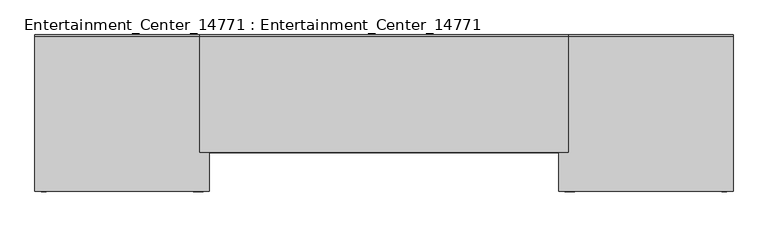
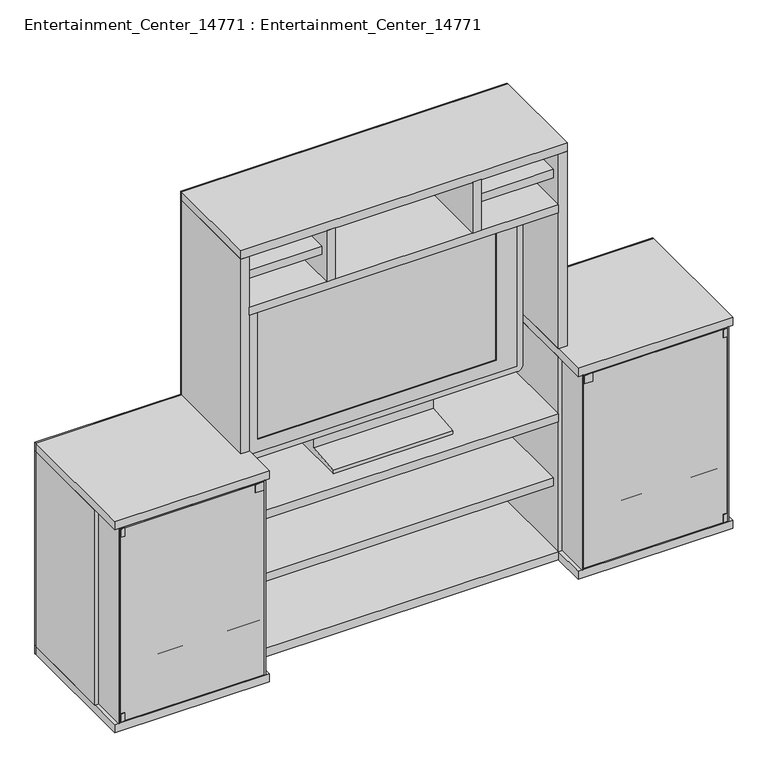
"""IFC4 building model written with IfcOpenShell, lengths in millimetres: furniture geometry, Entertainment_Center_14771 : Entertainment_Center_14771."""

from ifc_helpers import new_model, si_unit, point, frame, frame_2d, origin, origin_with_axes, place, context, project, spatial, polyline, circle_curve, ellipse_curve, trimmed, segment, composite_curve, outline, extrude, faceted_brep, source, transform, mapped, element, save
from ifc_brep_helpers import plane_surface, cylinder_surface, advanced_brep


def entertainment_center_14771_entertainment_center_14771_971748eb(model_context):
    return source(origin(), model_context, "Body", "SolidModel", [
        extrude(outline(polyline([(3.8418696, 537.2), (53.8418696, 537.2), (103.8418696, 457.2), (-96.1581304, 457.2), (-96.1581304, 467.2), (3.8418696, 477.2), (3.8418696, 537.2)])), frame((-176.4901536, 0.0, 0.0), z_axis=(1.0, 0.0, 0.0), x_axis=(0.0, 1.0, 0.0)), (0.0, 0.0, 1.0), 352.9803073),
        faceted_brep([(412.9803073, -14.1581304, 1014.3392838), (-412.9803073, -14.1581304, 1014.3392838), (-412.9803073, -14.1581304, 537.2), (412.9803073, -14.1581304, 537.2), (-352.9803073, -14.1581304, 974.3392838), (352.9803073, -14.1581304, 974.3392838), (352.9803073, -14.1581304, 577.2), (-352.9803073, -14.1581304, 577.2), (412.9803073, 3.8418696, 1014.3392838), (412.9803073, 3.8418696, 537.2), (-412.9803073, 3.8418696, 537.2), (-412.9803073, 3.8418696, 1014.3392838), (-352.9803073, -11.1581304, 974.3392838), (-352.9803073, -11.1581304, 577.2), (352.9803073, -11.1581304, 577.2), (352.9803073, -11.1581304, 974.3392838)], [[[0, 1, 2, 3], [4, 5, 6, 7]], [[8, 9, 10, 11]], [[1, 0, 8, 11]], [[2, 1, 11, 10]], [[3, 2, 10, 9]], [[0, 3, 9, 8]], [[12, 13, 14, 15]], [[12, 15, 5, 4]], [[15, 14, 6, 5]], [[14, 13, 7, 6]], [[13, 12, 4, 7]]]),
        extrude(outline(composite_curve([segment(polyline([(1034.3392838, 417.9803073), (1034.3392838, -417.9803073)]), True, "CONTINUOUS"), segment(trimmed(circle_curve(frame_2d((1019.3392838, -417.9803073)), 15.0), [point((1034.3392838, -417.9803073))], [point((1019.3392838, -432.9803073))], False, "CARTESIAN"), True, "CONTINUOUS"), segment(polyline([(1019.3392838, -432.9803073), (532.2, -432.9803073)]), True, "CONTINUOUS"), segment(trimmed(circle_curve(frame_2d((532.2, -417.9803073)), 15.0), [point((532.2, -432.9803073))], [point((517.2, -417.9803073))], False, "CARTESIAN"), True, "CONTINUOUS"), segment(polyline([(517.2, -417.9803073), (517.2, 417.9803073)]), True, "CONTINUOUS"), segment(trimmed(circle_curve(frame_2d((532.2, 417.9803073)), 15.0), [point((517.2, 417.9803073))], [point((532.2, 432.9803073))], False, "CARTESIAN"), True, "CONTINUOUS"), segment(polyline([(532.2, 432.9803073), (1019.3392838, 432.9803073)]), True, "CONTINUOUS"), segment(trimmed(circle_curve(frame_2d((1019.3392838, 417.9803073)), 15.0), [point((1019.3392838, 432.9803073))], [point((1034.3392838, 417.9803073))], False, "CARTESIAN"), True, "CONTINUOUS")], self_intersect=False), holes=[polyline([(1014.3392838, 412.9803073), (537.2, 412.9803073), (537.2, -412.9803073), (1014.3392838, -412.9803073), (1014.3392838, 412.9803073)])]), frame((0.0, -11.1581304, 0.0), z_axis=(0.0, 1.0, 0.0), x_axis=(0.0, 0.0, 1.0)), (0.0, 0.0, 1.0), 15.0),
        advanced_brep(
        [(-412.9803073, 3.8418696, 537.2), (412.9803073, 3.8418696, 537.2), (412.9803073, 3.8418696, 1014.3392838), (-412.9803073, 3.8418696, 1014.3392838), (302.9803073, 113.8418696, 537.2), (-302.9803073, 113.8418696, 537.2), (-302.9803073, 113.8418696, 904.3392838), (302.9803073, 113.8418696, 904.3392838)],
        [
            (0, 1),
            (1, 2),
            (2, 3),
            (3, 0),
            (4, 5),
            (5, 6),
            (6, 7),
            (7, 4),
            (0, 5, circle_curve(frame((-302.9803073, 3.8418696, 537.2), z_axis=(0.0, 0.0, -1.0), x_axis=(-1.0, 0.0, 0.0)), 110.0)),
            (4, 1, circle_curve(frame((302.9803073, 3.8418696, 537.2), z_axis=(0.0, 0.0, -1.0), x_axis=(1.0, 0.0, 0.0)), 110.0)),
            (7, 2, ellipse_curve(frame((302.9803073, 3.8418696, 904.3392838), z_axis=(0.7071067811865475, 0.0, -0.7071067811865475), x_axis=(0.7071067811865474, 0.0, 0.7071067811865476)), 155.5634919, 110.0)),
            (6, 3, ellipse_curve(frame((-302.9803073, 3.8418696, 904.3392838), z_axis=(0.7071067811865475, 0.0, 0.7071067811865475), x_axis=(-0.7071067811865476, 0.0, 0.7071067811865474)), 155.5634919, 110.0)),
        ],
        [
            plane_surface(frame((-412.9803073, 3.8418696, 1014.3392838), z_axis=(0.0, -1.0, 0.0), x_axis=(-1.0, 0.0, 0.0))),
            plane_surface(frame((-412.9803073, 113.8418696, 1014.3392838), z_axis=(0.0, 1.0, 0.0), x_axis=(1.0, 0.0, 0.0))),
            plane_surface(frame((-412.9803073, 3.8418696, 537.2), z_axis=(0.0, 0.0, -1.0), x_axis=(0.0, 1.0, 0.0))),
            cylinder_surface(frame((302.9803073, 3.8418696, 537.2), z_axis=(0.0, 0.0, 1.0), x_axis=(1.0, 0.0, 0.0)), 110.0),
            cylinder_surface(frame((412.9803073, 3.8418696, 904.3392838), z_axis=(-1.0, 0.0, 0.0), x_axis=(0.0, 0.0, 1.0)), 110.0),
            cylinder_surface(frame((-302.9803073, 3.8418696, 1014.3392838), z_axis=(0.0, 0.0, -1.0), x_axis=(-1.0, 0.0, 0.0)), 110.0),
        ],
        [
            (0, [[1, 2, 3, 4]]),
            (1, [[5, 6, 7, 8]]),
            (2, [[-1, 9, -5, 10]]),
            (3, [[11, -2, -10, -8]]),
            (4, [[-11, -7, 12, -3]]),
            (5, [[-12, -6, -9, -4]]),
        ],
    ),
        extrude(outline(polyline([(468.3125, -254.0), (468.3125, -152.4), (471.4875, -152.4), (471.4875, -254.0), (468.3125, -254.0)])), frame((0.0, 0.0, 25.4), z_axis=(0.0, 0.0, 1.0), x_axis=(1.0, 0.0, 0.0)), (0.0, 0.0, 1.0), 609.6),
        extrude(outline(polyline([(474.0377403, -254.8079035), (474.0377403, -253.9978359), (499.2974238, -253.9978359), (499.2974238, -254.8079035), (474.0377403, -254.8079035)])), frame((0.0, 0.0, 606.4088319), z_axis=(0.0, 0.0, 1.0), x_axis=(1.0, 0.0, 0.0)), (0.0, 0.0, 1.0), 25.4),
        extrude(outline(polyline([(885.1998705, -253.9978359), (896.9429841, -253.9978359), (896.9429841, -250.8228359), (885.1998705, -250.8228359), (885.1998705, -250.0409988), (897.6232054, -250.0409988), (897.6232054, -254.7888134), (885.1998705, -254.7888134), (885.1998705, -253.9978359)])), frame((0.0, 0.0, 28.43226), z_axis=(0.0, 0.0, 1.0), x_axis=(1.0, 0.0, 0.0)), (0.0, 0.0, 1.0), 25.4),
        extrude(outline(polyline([(885.1998705, -253.9978359), (896.9429841, -253.9978359), (896.9429841, -250.8228359), (885.1998705, -250.8228359), (885.1998705, -250.0409988), (897.6232054, -250.0409988), (897.6232054, -254.7888134), (885.1998705, -254.7888134), (885.1998705, -253.9978359)])), frame((0.0, 0.0, 606.4088319), z_axis=(0.0, 0.0, 1.0), x_axis=(1.0, 0.0, 0.0)), (0.0, 0.0, 1.0), 25.4),
        extrude(outline(polyline([(900.1125, -254.0), (900.1125, -152.4), (903.2875, -152.4), (903.2875, -254.0), (900.1125, -254.0)])), frame((0.0, 0.0, 25.4), z_axis=(0.0, 0.0, 1.0), x_axis=(1.0, 0.0, 0.0)), (0.0, 0.0, 1.0), 609.6),
        extrude(outline(polyline([(474.0377403, -250.8228359), (896.9429841, -250.8228359), (896.9429841, -253.9978359), (474.0377403, -253.9978359), (474.0377403, -250.8228359)])), frame((0.0, 0.0, 28.43226), z_axis=(0.0, 0.0, 1.0), x_axis=(1.0, 0.0, 0.0)), (0.0, 0.0, 1.0), 603.3765719),
        extrude(outline(polyline([(-474.0377403, -254.8079035), (-499.2974238, -254.8079035), (-499.2974238, -253.9978359), (-474.0377403, -253.9978359), (-474.0377403, -254.8079035)])), frame((0.0, 0.0, 606.4088319), z_axis=(0.0, 0.0, 1.0), x_axis=(1.0, 0.0, 0.0)), (0.0, 0.0, 1.0), 25.4),
        extrude(outline(polyline([(-885.1998705, -253.9978359), (-885.1998705, -254.7888134), (-897.6232054, -254.7888134), (-897.6232054, -250.0409988), (-885.1998705, -250.0409988), (-885.1998705, -250.8228359), (-896.9429841, -250.8228359), (-896.9429841, -253.9978359), (-885.1998705, -253.9978359)])), frame((0.0, 0.0, 28.43226), z_axis=(0.0, 0.0, 1.0), x_axis=(1.0, 0.0, 0.0)), (0.0, 0.0, 1.0), 25.4),
        extrude(outline(polyline([(-885.1998705, -253.9978359), (-885.1998705, -254.7888134), (-897.6232054, -254.7888134), (-897.6232054, -250.0409988), (-885.1998705, -250.0409988), (-885.1998705, -250.8228359), (-896.9429841, -250.8228359), (-896.9429841, -253.9978359), (-885.1998705, -253.9978359)])), frame((0.0, 0.0, 606.4088319), z_axis=(0.0, 0.0, 1.0), x_axis=(1.0, 0.0, 0.0)), (0.0, 0.0, 1.0), 25.4),
        extrude(outline(polyline([(-468.3125, -254.0), (-471.4875, -254.0), (-471.4875, -152.4), (-468.3125, -152.4), (-468.3125, -254.0)])), frame((0.0, 0.0, 25.4), z_axis=(0.0, 0.0, 1.0), x_axis=(1.0, 0.0, 0.0)), (0.0, 0.0, 1.0), 609.6),
        extrude(outline(polyline([(-900.1125, -254.0), (-903.2875, -254.0), (-903.2875, -152.4), (-900.1125, -152.4), (-900.1125, -254.0)])), frame((0.0, 0.0, 25.4), z_axis=(0.0, 0.0, 1.0), x_axis=(1.0, 0.0, 0.0)), (0.0, 0.0, 1.0), 609.6),
        extrude(outline(polyline([(-474.0377403, -250.8228359), (-474.0377403, -253.9978359), (-896.9429841, -253.9978359), (-896.9429841, -250.8228359), (-474.0377403, -250.8228359)])), frame((0.0, 0.0, 28.43226), z_axis=(0.0, 0.0, 1.0), x_axis=(1.0, 0.0, 0.0)), (0.0, 0.0, 1.0), 603.3765719),
        extrude(outline(polyline([(1295.4, 482.6), (1295.4, -482.6), (1270.0, -482.6), (660.4, -482.6), (660.4, -914.4), (635.0, -914.4), (25.4, -914.4), (0.0, -914.4), (0.0, 914.4), (25.4, 914.4), (635.0, 914.4), (660.4, 914.4), (660.4, 482.6), (1270.0, 482.6), (1295.4, 482.6)])), frame((0.0, 152.4, 0.0), z_axis=(0.0, 1.0, 0.0), x_axis=(0.0, 0.0, 1.0)), (0.0, 0.0, 1.0), 3.175),
        extrude(outline(polyline([(457.2, 152.4), (457.2, -127.0), (228.6, -127.0), (228.6, 152.4), (457.2, 152.4)])), frame((0.0, 0.0, 1180.3892838), z_axis=(0.0, 0.0, 1.0), x_axis=(1.0, 0.0, 0.0)), (0.0, 0.0, 1.0), 25.4),
        extrude(outline(polyline([(-228.6, 152.4), (-228.6, -127.0), (-457.2, -127.0), (-457.2, 152.4), (-228.6, 152.4)])), frame((0.0, 0.0, 1180.3892838), z_axis=(0.0, 0.0, 1.0), x_axis=(1.0, 0.0, 0.0)), (0.0, 0.0, 1.0), 25.4),
        extrude(outline(polyline([(457.2, 152.4), (457.2, -127.0), (-457.2, -127.0), (-457.2, 152.4), (457.2, 152.4)])), frame((0.0, 0.0, 215.9), z_axis=(0.0, 0.0, 1.0), x_axis=(1.0, 0.0, 0.0)), (0.0, 0.0, 1.0), 25.4),
        extrude(outline(polyline([(228.6, 152.4), (228.6, -152.4), (203.2, -152.4), (203.2, 152.4), (228.6, 152.4)])), frame((0.0, 0.0, 1110.5392838), z_axis=(0.0, 0.0, 1.0), x_axis=(1.0, 0.0, 0.0)), (0.0, 0.0, 1.0), 159.4607162),
        extrude(outline(polyline([(-203.2, 152.4), (-203.2, -152.4), (-228.6, -152.4), (-228.6, 152.4), (-203.2, 152.4)])), frame((0.0, 0.0, 1110.5392838), z_axis=(0.0, 0.0, 1.0), x_axis=(1.0, 0.0, 0.0)), (0.0, 0.0, 1.0), 159.4607162),
        extrude(outline(polyline([(889.0, 152.4), (889.0, -254.0), (482.6, -254.0), (482.6, 152.4), (889.0, 152.4)])), frame((0.0, 0.0, 482.6), z_axis=(0.0, 0.0, 1.0), x_axis=(1.0, 0.0, 0.0)), (0.0, 0.0, 1.0), 25.4),
        extrude(outline(polyline([(889.0, 152.4), (889.0, -254.0), (482.6, -254.0), (482.6, 152.4), (889.0, 152.4)])), frame((0.0, 0.0, 330.2), z_axis=(0.0, 0.0, 1.0), x_axis=(1.0, 0.0, 0.0)), (0.0, 0.0, 1.0), 25.4),
        extrude(outline(polyline([(889.0, 152.4), (889.0, -254.0), (482.6, -254.0), (482.6, 152.4), (889.0, 152.4)])), frame((0.0, 0.0, 177.8), z_axis=(0.0, 0.0, 1.0), x_axis=(1.0, 0.0, 0.0)), (0.0, 0.0, 1.0), 25.4),
        extrude(outline(polyline([(-482.6, 152.4), (-482.6, -254.0), (-889.0, -254.0), (-889.0, 152.4), (-482.6, 152.4)])), frame((0.0, 0.0, 482.6), z_axis=(0.0, 0.0, 1.0), x_axis=(1.0, 0.0, 0.0)), (0.0, 0.0, 1.0), 25.4),
        extrude(outline(polyline([(-482.6, 152.4), (-482.6, -254.0), (-889.0, -254.0), (-889.0, 152.4), (-482.6, 152.4)])), frame((0.0, 0.0, 330.2), z_axis=(0.0, 0.0, 1.0), x_axis=(1.0, 0.0, 0.0)), (0.0, 0.0, 1.0), 25.4),
        extrude(outline(polyline([(-482.6, 152.4), (-482.6, -254.0), (-889.0, -254.0), (-889.0, 152.4), (-482.6, 152.4)])), frame((0.0, 0.0, 177.8), z_axis=(0.0, 0.0, 1.0), x_axis=(1.0, 0.0, 0.0)), (0.0, 0.0, 1.0), 25.4),
        extrude(outline(polyline([(457.2, 152.4), (457.2, -152.4), (-457.2, -152.4), (-457.2, 152.4), (457.2, 152.4)])), frame((0.0, 0.0, 1085.1392838), z_axis=(0.0, 0.0, 1.0), x_axis=(1.0, 0.0, 0.0)), (0.0, 0.0, 1.0), 25.4),
        extrude(outline(polyline([(482.6, 152.4), (482.6, -152.4), (-482.6, -152.4), (-482.6, 152.4), (482.6, 152.4)])), frame((0.0, 0.0, 1270.0), z_axis=(0.0, 0.0, 1.0), x_axis=(1.0, 0.0, 0.0)), (0.0, 0.0, 1.0), 25.4),
        extrude(outline(polyline([(482.6, 152.4), (482.6, -152.4), (457.2, -152.4), (457.2, 152.4), (482.6, 152.4)])), frame((0.0, 0.0, 660.4), z_axis=(0.0, 0.0, 1.0), x_axis=(1.0, 0.0, 0.0)), (0.0, 0.0, 1.0), 609.6),
        extrude(outline(polyline([(-457.2, 152.4), (-457.2, -152.4), (-482.6, -152.4), (-482.6, 152.4), (-457.2, 152.4)])), frame((0.0, 0.0, 660.4), z_axis=(0.0, 0.0, 1.0), x_axis=(1.0, 0.0, 0.0)), (0.0, 0.0, 1.0), 609.6),
        extrude(outline(polyline([(457.2, 152.4), (457.2, -152.4), (-457.2, -152.4), (-457.2, 152.4), (457.2, 152.4)])), frame((0.0, 0.0, 431.8), z_axis=(0.0, 0.0, 1.0), x_axis=(1.0, 0.0, 0.0)), (0.0, 0.0, 1.0), 25.4),
        extrude(outline(polyline([(914.4, 152.4), (914.4, -254.0), (457.2, -254.0), (457.2, 152.4), (914.4, 152.4)])), frame((0.0, 0.0, 635.0), z_axis=(0.0, 0.0, 1.0), x_axis=(1.0, 0.0, 0.0)), (0.0, 0.0, 1.0), 25.4),
        extrude(outline(polyline([(-457.2, 152.4), (-457.2, -254.0), (-914.4, -254.0), (-914.4, 152.4), (-457.2, 152.4)])), frame((0.0, 0.0, 635.0), z_axis=(0.0, 0.0, 1.0), x_axis=(1.0, 0.0, 0.0)), (0.0, 0.0, 1.0), 25.4),
        extrude(outline(polyline([(482.6, 152.4), (482.6, -152.4), (457.2, -152.4), (457.2, 152.4), (482.6, 152.4)])), frame((0.0, 0.0, 25.4), z_axis=(0.0, 0.0, 1.0), x_axis=(1.0, 0.0, 0.0)), (0.0, 0.0, 1.0), 609.6),
        extrude(outline(polyline([(-457.2, 152.4), (-457.2, -152.4), (-482.6, -152.4), (-482.6, 152.4), (-457.2, 152.4)])), frame((0.0, 0.0, 25.4), z_axis=(0.0, 0.0, 1.0), x_axis=(1.0, 0.0, 0.0)), (0.0, 0.0, 1.0), 609.6),
        extrude(outline(polyline([(914.4, 152.4), (914.4, -152.4), (889.0, -152.4), (889.0, 152.4), (914.4, 152.4)])), frame((0.0, 0.0, 25.4), z_axis=(0.0, 0.0, 1.0), x_axis=(1.0, 0.0, 0.0)), (0.0, 0.0, 1.0), 609.6),
        extrude(outline(polyline([(-889.0, 152.4), (-889.0, -152.4), (-914.4, -152.4), (-914.4, 152.4), (-889.0, 152.4)])), frame((0.0, 0.0, 25.4), z_axis=(0.0, 0.0, 1.0), x_axis=(1.0, 0.0, 0.0)), (0.0, 0.0, 1.0), 609.6),
        extrude(outline(polyline([(914.4, 152.4), (914.4, -254.0), (457.2, -254.0), (457.2, -152.4), (-457.2, -152.4), (-457.2, -254.0), (-914.4, -254.0), (-914.4, 152.4), (914.4, 152.4)])), origin_with_axes(), (0.0, 0.0, 1.0), 25.4),
    ])


if __name__ == "__main__":
    model = new_model("IFC4")
    model_context = context("Model", 3, world=origin())
    ifc_project = project(units=[si_unit("LENGTHUNIT", "METRE", prefix="MILLI")], contexts=[model_context])
    site = spatial("IfcSite", under=ifc_project)
    building = spatial("IfcBuilding", under=site)
    placement = place(None, origin())
    entertainment_center_14771_entertainment_center_14771_shape = entertainment_center_14771_entertainment_center_14771_971748eb(model_context)
    element("IfcFurniture", 1, ObjectType="Entertainment_Center_14771 : Entertainment_Center_14771", at=placement, inside=building, context=model_context, shape_type="MappedRepresentation", body=[
        mapped(entertainment_center_14771_entertainment_center_14771_shape, transform((0.0, 0.0, 0.0), x_axis=(1.0, 0.0, 0.0), y_axis=(0.0, 1.0, 0.0), z_axis=(0.0, 0.0, 1.0))),
    ])
    save(model, "model.ifc")

# Revit data of these elements
# Element 1 (IfcFurniture, "Entertainment_Center_14771 : Entertainment_Center_14771")
#   Materials on its faces: "Cherry", "Stainless Steel, Polished", "Glass 2", "TV - Black", "TV - Glass", "TV - Screen"
# Materials
#   "Cherry": class "Wood", colour RGB 154 107 61, transparency 0, Description = "Prunus Serotina", Cost = 0
#   "Stainless Steel, Polished": class "Metal", colour RGB 120 120 120, transparency 0, Description = "Stainless Steel 18/8, polished finish", Cost = 0
#   "Glass 2": class "Glass", colour RGB 164 164 255, transparency 0.75, Cost = 0
#   "TV - Black": class "Miscellaneous", colour RGB 49 49 49, transparency 0
#   "TV - Glass": class "Miscellaneous", colour RGB 157 157 157, transparency 0.9
#   "TV - Screen": class "Miscellaneous", colour RGB 0 0 0, transparency 0
